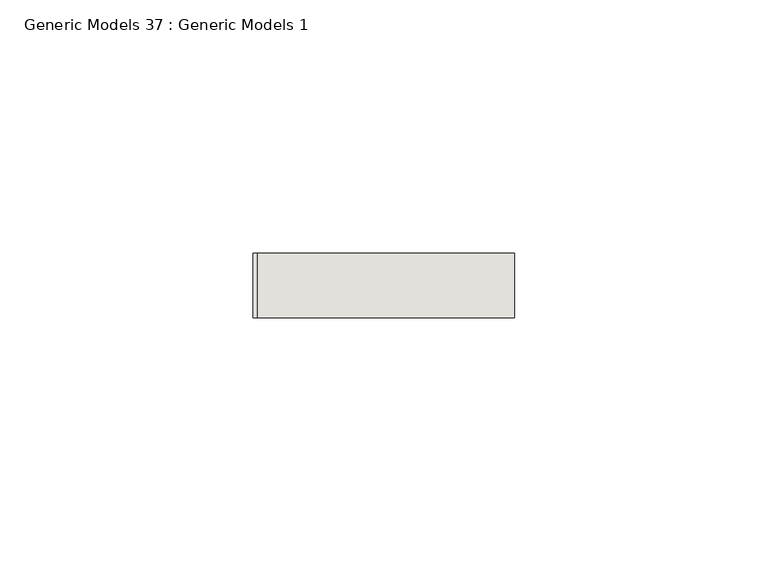
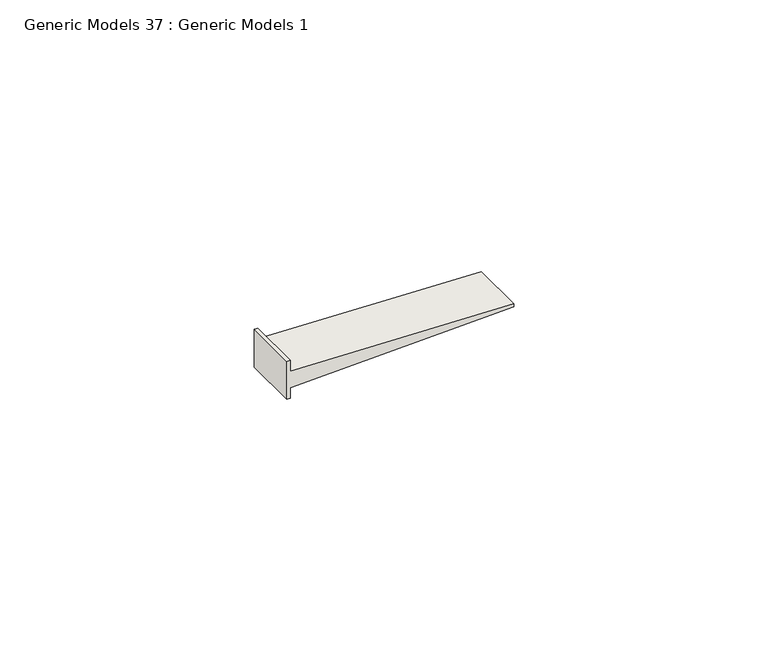
"""IFC4 building model written with IfcOpenShell, lengths in millimetres: wall geometry, Generic Models 37 : Generic Models 1."""

from ifc_helpers import new_model, si_unit, frame, origin, place, context, project, spatial, polyline, outline, extrude, source, transform, mapped, element, save


def generic_models_37_generic_models_1_916dd7c6(model_context):
    return source(origin(), model_context, "Body", "SweptSolid", [
        extrude(outline(polyline([(2409.6091, 49675.25625), (2400.5159, 49675.25625), (2400.5159, 49676.05), (2403.0657636, 49676.05), (2404.6631527, 49726.85), (2405.4618473, 49726.85), (2407.0592364, 49676.05), (2409.6091, 49676.05), (2409.6091, 49675.25625)])), frame((0.0, 565.15, 0.0), z_axis=(0.0, 1.0, 0.0), x_axis=(0.0, 0.0, 1.0)), (0.0, 0.0, 1.0), 12.7),
    ])


if __name__ == "__main__":
    model = new_model("IFC4")
    model_context = context("Model", 3, world=origin())
    ifc_project = project(units=[si_unit("LENGTHUNIT", "METRE", prefix="MILLI")], contexts=[model_context])
    site = spatial("IfcSite", under=ifc_project)
    building = spatial("IfcBuilding", under=site)
    placement = place(None, origin())
    generic_models_37_generic_models_1_shape = generic_models_37_generic_models_1_916dd7c6(model_context)
    element("IfcWall", 1, ObjectType="Generic Models 37 : Generic Models 1", at=placement, inside=building, context=model_context, shape_type="MappedRepresentation", body=[
        mapped(generic_models_37_generic_models_1_shape, transform((0.0, 0.0, 0.0), x_axis=(1.0, 0.0, 0.0), y_axis=(0.0, 1.0, 0.0), z_axis=(0.0, 0.0, 1.0))),
    ])
    save(model, "model.ifc")

# Revit data of these elements
# Element 1 (IfcWall, "Generic Models 37 : Generic Models 1")
#   Materials on its faces: "ATTACH GYPSUM BOARD TO STUDS AND NOT TO TOP TRACK"
# Materials
#   "ATTACH GYPSUM BOARD TO STUDS AND NOT TO TOP TRACK": class "Generic", colour RGB 48 48 48, transparency 0, Cost = 0
